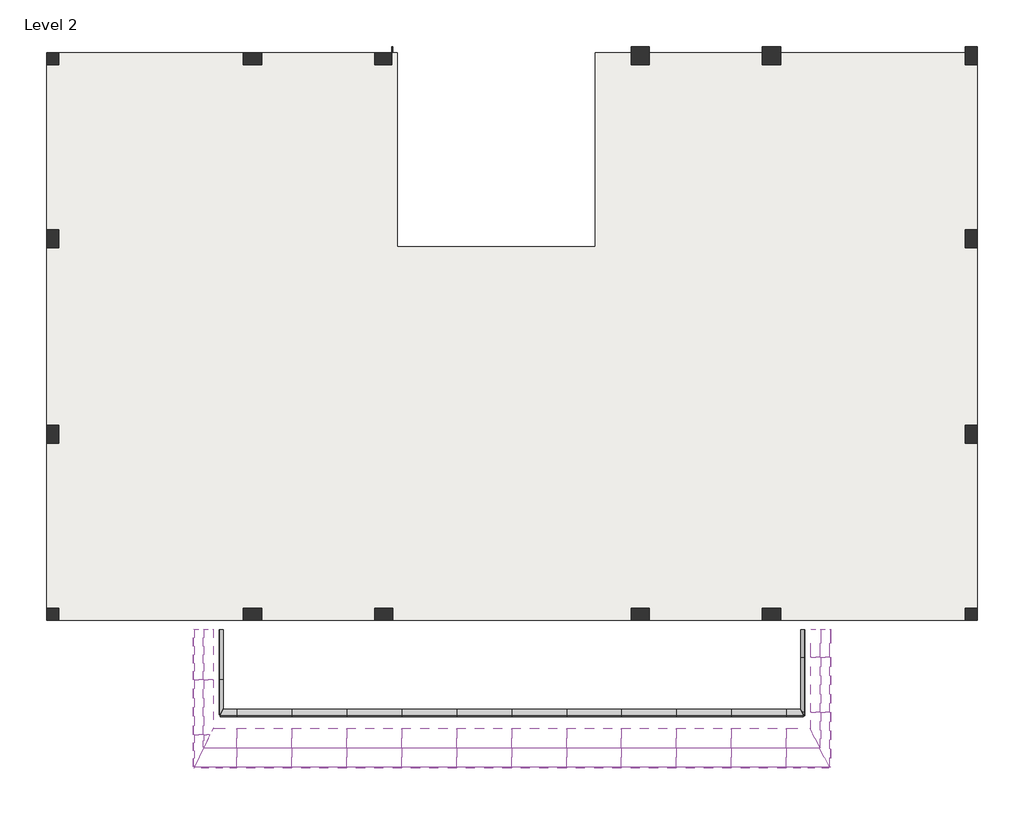
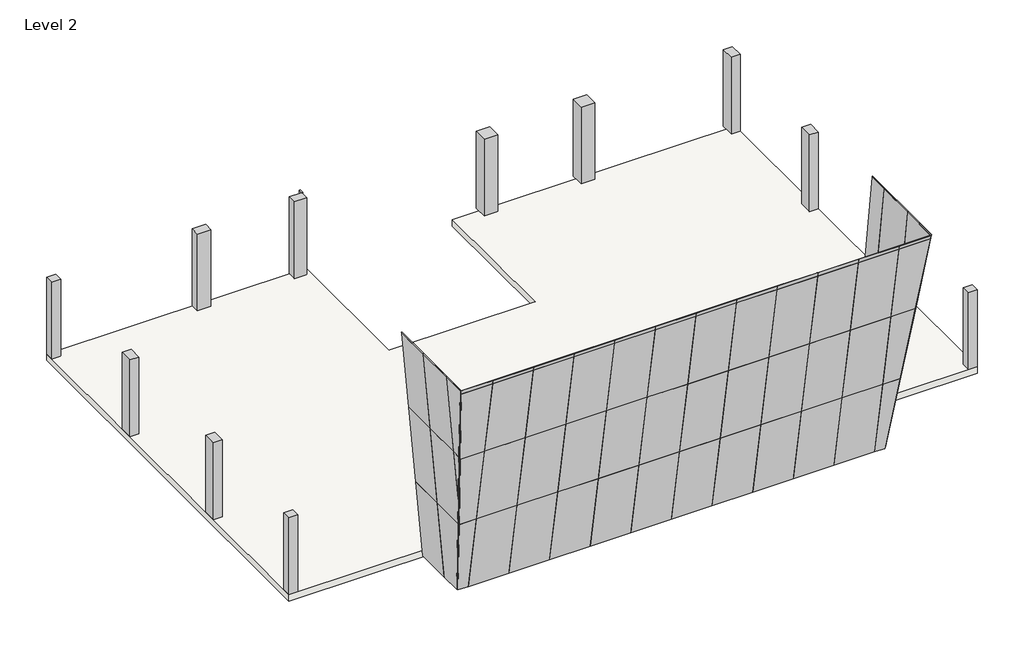
# One storey: 71 plates, 16 columns, 1 slab.
"""IFC4 building model written with IfcOpenShell, lengths in millimetres."""

import ifcopenshell
import ifcopenshell.guid

model = None  # the IFC model being written
_history = None  # IfcOwnerHistory: only IFC2X3 demands one
_inside = {}  # id of a spatial element -> (the spatial element, [elements in it])
_under = {}  # id of a project, library or spatial element -> (it, [spatial elements below it])
_declared = {}  # id of a project -> (the project, [libraries it declares])
_typed = {}  # id of a type object -> (the type object, [elements of that type])
_made_of = {}  # id of a material, layer set ... -> (it, [elements and type objects made of it])


def new_model(schema):
    """Start an empty IFC model of exactly this schema.

    Asked for "IFC4X3", IfcOpenShell would pick the latest addendum, in which some entities
    have other attributes; the version numbers below select the first issue.
    IFC2X3 requires an IfcOwnerHistory on every rooted entity: one is made here for all.
    """
    global model, _history
    if schema == "IFC4X3":
        model = ifcopenshell.file(schema_version=(4, 3, 0, 0))
    else:
        model = ifcopenshell.file(schema=schema)
    _inside.clear()
    _under.clear()
    _declared.clear()
    _typed.clear()
    _made_of.clear()
    _history = None
    if model.schema == "IFC2X3":
        org = make("IfcOrganization", Name="unknown")
        user = make(
            "IfcPersonAndOrganization",
            ThePerson=make("IfcPerson", FamilyName="unknown"),
            TheOrganization=org,
        )
        app = make(
            "IfcApplication",
            ApplicationDeveloper=org,
            Version="unknown",
            ApplicationFullName="unknown",
            ApplicationIdentifier="unknown",
        )
        _history = make(
            "IfcOwnerHistory",
            OwningUser=user,
            OwningApplication=app,
            ChangeAction="ADDED",
            CreationDate=0,
        )
    return model


def make(cls, **values):
    """One entity of the class cls with the attributes given. An attribute that is None is left unset."""
    return model.create_entity(
        cls, **{name: value for name, value in values.items() if value is not None}
    )


def rooted(cls, **values):
    """An entity with a GlobalId (a new one), such as an element, a storey or a relation."""
    return make(cls, GlobalId=ifcopenshell.guid.new(), OwnerHistory=_history, **values)


def si_unit(unit_type, name, prefix=None):
    """IfcSIUnit, for example si_unit("LENGTHUNIT", "METRE", prefix="MILLI")."""
    return make("IfcSIUnit", UnitType=unit_type, Prefix=prefix, Name=name)


def assignment(units):
    """IfcUnitAssignment: the units of a project."""
    return None if units is None else make("IfcUnitAssignment", Units=units)


def point(xyz):
    """IfcCartesianPoint."""
    return None if xyz is None else make("IfcCartesianPoint", Coordinates=xyz)


def direction(xyz):
    """IfcDirection."""
    return None if xyz is None else make("IfcDirection", DirectionRatios=xyz)


def frame(location, z_axis=None, x_axis=None):
    """IfcAxis2Placement3D, a coordinate frame: its origin and axes. An axis left out is left unset."""
    return make(
        "IfcAxis2Placement3D",
        Location=point(location),
        Axis=direction(z_axis),
        RefDirection=direction(x_axis),
    )


def origin():
    """The frame at (0, 0, 0) with its axes left unset."""
    return frame((0.0, 0.0, 0.0))


def origin_with_axes():
    """The frame at (0, 0, 0) with the z axis (0, 0, 1) and the x axis (1, 0, 0) written out."""
    return frame((0.0, 0.0, 0.0), z_axis=(0.0, 0.0, 1.0), x_axis=(1.0, 0.0, 0.0))


def place(relative_to, where):
    """IfcLocalPlacement: puts the frame where relative to a parent placement (None: the world)."""
    return make(
        "IfcLocalPlacement", PlacementRelTo=relative_to, RelativePlacement=where
    )


def context(
    kind, dimensions, precision=None, world=None, true_north=None, identifier=None
):
    """IfcGeometricRepresentationContext, for example the 3D "Model" context."""
    return make(
        "IfcGeometricRepresentationContext",
        ContextIdentifier=identifier,
        ContextType=kind,
        CoordinateSpaceDimension=dimensions,
        Precision=precision,
        WorldCoordinateSystem=world,
        TrueNorth=true_north,
    )


def project(units=None, contexts=None):
    """IfcProject with its units and contexts."""
    return rooted(
        "IfcProject",
        Name="project",
        RepresentationContexts=contexts,
        UnitsInContext=assignment(units),
    )


def spatial(cls, under=None, at=None, **own):
    """A site, building, storey or space (cls), placed at a placement, below another one or the project."""
    s = rooted(cls, ObjectPlacement=at, **own)
    if under is not None:
        _under.setdefault(under.id(), (under, []))[1].append(s)
    return s


def polyline(points):
    """IfcPolyline through the points."""
    return make("IfcPolyline", Points=[point(p) for p in points])


def outline(outer, holes=None, kind="AREA"):
    """IfcArbitraryClosedProfileDef: a profile drawn as a closed curve; with holes, ...WithVoids."""
    if holes is None:
        return make("IfcArbitraryClosedProfileDef", ProfileType=kind, OuterCurve=outer)
    return make(
        "IfcArbitraryProfileDefWithVoids",
        ProfileType=kind,
        OuterCurve=outer,
        InnerCurves=holes,
    )


def extrude(swept, where, along, depth):
    """IfcExtrudedAreaSolid: the profile swept, set in the frame where, extruded along a direction by depth."""
    return make(
        "IfcExtrudedAreaSolid",
        SweptArea=swept,
        Position=where,
        ExtrudedDirection=direction(along),
        Depth=depth,
    )


def shape(context_of_items, identifier, shape_type, items):
    """IfcShapeRepresentation: the items that make up one representation, for example the "Body"."""
    return make(
        "IfcShapeRepresentation",
        ContextOfItems=context_of_items,
        RepresentationIdentifier=identifier,
        RepresentationType=shape_type,
        Items=items,
    )


def source(mapping_origin, context_of_items, identifier, shape_type, items):
    """IfcRepresentationMap: a shape defined once, which mapped items show again and again."""
    return make(
        "IfcRepresentationMap",
        MappingOrigin=mapping_origin,
        MappedRepresentation=shape(context_of_items, identifier, shape_type, items),
    )


def transform(
    local_origin,
    x_axis=None,
    y_axis=None,
    z_axis=None,
    scale=None,
    scale2=None,
    scale3=None,
    uniform=True,
):
    """IfcCartesianTransformationOperator3D, or its non-uniform kind. x_axis, y_axis, z_axis: its Axis1, 2, 3."""
    if uniform:
        return make(
            "IfcCartesianTransformationOperator3D",
            Axis1=direction(x_axis),
            Axis2=direction(y_axis),
            LocalOrigin=point(local_origin),
            Scale=scale,
            Axis3=direction(z_axis),
        )
    return make(
        "IfcCartesianTransformationOperator3DnonUniform",
        Axis1=direction(x_axis),
        Axis2=direction(y_axis),
        LocalOrigin=point(local_origin),
        Scale=scale,
        Axis3=direction(z_axis),
        Scale2=scale2,
        Scale3=scale3,
    )


def mapped(mapping_source, mapping_target):
    """IfcMappedItem: shows the shape of a source again, moved by a transform."""
    return make(
        "IfcMappedItem", MappingSource=mapping_source, MappingTarget=mapping_target
    )


def made_of(thing, what):
    """Note that an element or type object is made of a material, layer set ...; save() writes the relation."""
    if what is not None:
        _made_of.setdefault(what.id(), (what, []))[1].append(thing)
    return thing


def element(
    cls,
    number,
    at=None,
    inside=None,
    cuts=None,
    type_object=None,
    material=None,
    context=None,
    identifier="Body",
    shape_type=None,
    held_by="IfcProductDefinitionShape",
    body=None,
    shapes=None,
    **own,
):
    """One element of the class cls, such as IfcWall. Its Tag is "e" and its number.

    at: its placement. inside: the storey or other place that contains it. cuts: it is an
    opening in that element (IfcRelVoidsElement). A single representation is given by context,
    identifier, shape_type and body (its items); several are given by shapes. held_by: the class
    of the entity that holds the representations. save() writes the other relations.
    """
    e = rooted(cls, Tag="e%d" % number, ObjectPlacement=at, **own)
    if body is not None:
        shapes = [shape(context, identifier, shape_type, body)]
    if shapes is not None:
        e.Representation = make(held_by, Representations=shapes)
    if inside is not None:
        _inside.setdefault(inside.id(), (inside, []))[1].append(e)
    if cuts is not None:
        rooted(
            "IfcRelVoidsElement", RelatingBuildingElement=cuts, RelatedOpeningElement=e
        )
    if type_object is not None:
        _typed.setdefault(type_object.id(), (type_object, []))[1].append(e)
    return made_of(e, material)


def aggregate(whole, parts):
    """IfcRelAggregates: a whole, such as a stair, and the parts it consists of."""
    return rooted("IfcRelAggregates", RelatingObject=whole, RelatedObjects=parts)


def save(model, path):
    """Write the relations noted so far, then the file.

    IfcRelAggregates (storeys below a building ...), IfcRelContainedInSpatialStructure (elements
    in a storey), IfcRelDefinesByType, IfcRelAssociatesMaterial and IfcRelDeclares: one each for
    every whole, place, type object, material and project.
    """
    for whole, parts in _under.values():
        aggregate(whole, parts)
    for where, things in _inside.values():
        rooted(
            "IfcRelContainedInSpatialStructure",
            RelatedElements=things,
            RelatingStructure=where,
        )
    for kind, things in _typed.values():
        rooted("IfcRelDefinesByType", RelatedObjects=things, RelatingType=kind)
    for what, things in _made_of.values():
        rooted("IfcRelAssociatesMaterial", RelatedObjects=things, RelatingMaterial=what)
    for by, libraries in _declared.values():
        rooted("IfcRelDeclares", RelatingContext=by, RelatedDefinitions=libraries)
    model.write(path)


def system_panel_glazed_2e91cb65(model_context):
    return source(origin(), model_context, "Body", "SweptSolid", [
        extrude(outline(polyline([(838.2000002, -44.45), (-838.2000002, -44.45), (-838.2000002, -19.05), (838.2000002, -19.05), (838.2000002, -44.45)])), origin_with_axes(), (0.0, 0.0, 1.0), 3657.6),
    ])


def system_panel_glazed_41c8569a(model_context):
    return source(origin(), model_context, "Body", "SweptSolid", [
        extrude(outline(polyline([(3054.1438606, -268.2393521), (0.0, 268.2393521), (3054.1438606, 268.2393521), (3054.1438606, -268.2393521)])), frame((0.0, -44.45, 0.0), z_axis=(0.0, 1.0, 0.0), x_axis=(0.0, 0.0, 1.0)), (0.0, 0.0, 1.0), 25.4),
    ])


def system_panel_glazed_2bad594a(model_context):
    return source(origin(), model_context, "Body", "SweptSolid", [
        extrude(outline(polyline([(0.0, -797.3917397), (0.0, 154.912342), (3657.6, 797.3917397), (3657.6, -797.3917397), (0.0, -797.3917397)])), frame((0.0, -44.45, 0.0), z_axis=(0.0, 1.0, 0.0), x_axis=(0.0, 0.0, 1.0)), (0.0, 0.0, 1.0), 25.4),
    ])


def system_panel_glazed_87679f4c(model_context):
    return source(origin(), model_context, "Body", "SweptSolid", [
        extrude(outline(polyline([(0.0, -914.4), (0.0, 680.3834794), (1332.2432262, 914.4), (3657.6, 914.4), (3657.6, -914.4), (0.0, -914.4)])), frame((0.0, -44.45, 0.0), z_axis=(0.0, 1.0, 0.0), x_axis=(0.0, 0.0, 1.0)), (0.0, 0.0, 1.0), 25.4),
    ])


def system_panel_glazed_96c5221b(model_context):
    return source(origin(), model_context, "Body", "SweptSolid", [
        extrude(outline(polyline([(0.0, -204.2314386), (2325.3567738, 204.2314386), (2325.3567738, -204.2314386), (0.0, -204.2314386)])), frame((0.0, -44.45, 0.0), z_axis=(0.0, 1.0, 0.0), x_axis=(0.0, 0.0, 1.0)), (0.0, 0.0, 1.0), 25.4),
    ])


def system_panel_glazed_1f34555f(model_context):
    return source(origin(), model_context, "Body", "SweptSolid", [
        extrude(outline(polyline([(914.4, -44.45), (-914.4, -44.45), (-914.4, -19.05), (914.4, -19.05), (914.4, -44.45)])), origin_with_axes(), (0.0, 0.0, 1.0), 3657.6),
    ])


def system_panel_glazed_ce152239(model_context):
    return source(origin(), model_context, "Body", "SweptSolid", [
        extrude(outline(polyline([(0.0, -525.4711374), (0.0, -117.0082603), (3657.6, 525.4711374), (3657.6, -525.4711374), (0.0, -525.4711374)])), frame((0.0, -44.45, 0.0), z_axis=(0.0, 1.0, 0.0), x_axis=(0.0, 0.0, 1.0)), (0.0, 0.0, 1.0), 25.4),
    ])


def system_panel_glazed_8b4ddac8(model_context):
    return source(origin(), model_context, "Body", "SweptSolid", [
        extrude(outline(polyline([(838.2000002, -44.45), (-838.2000002, -44.45), (-838.2000002, -19.05), (838.2000002, -19.05), (838.2000002, -44.45)])), origin_with_axes(), (0.0, 0.0, 1.0), 41.9143134),
    ])


def system_panel_glazed_7f82afe2(model_context):
    return source(origin(), model_context, "Body", "SweptSolid", [
        extrude(outline(polyline([(914.4, -44.45), (-914.4, -44.45), (-914.4, -19.05), (914.4, -19.05), (914.4, -44.45)])), origin_with_axes(), (0.0, 0.0, 1.0), 41.9143134),
    ])


def system_panel_glazed_3146f186(model_context):
    return source(origin(), model_context, "Body", "SweptSolid", [
        extrude(outline(polyline([(0.0, -529.1523878), (0.0, 521.789887), (41.9143134, 529.1523878), (41.9143134, -529.1523878), (0.0, -529.1523878)])), frame((0.0, -44.45, 0.0), z_axis=(0.0, 1.0, 0.0), x_axis=(0.0, 0.0, 1.0)), (0.0, 0.0, 1.0), 25.4),
    ])


def system_panel_glazed_f4345ae3(model_context):
    return source(origin(), model_context, "Body", "SweptSolid", [
        extrude(outline(polyline([(914.4, -44.45), (-914.4, -44.45), (-914.4, -19.05), (914.4, -19.05), (914.4, -44.45)])), origin_with_axes(), (0.0, 0.0, 1.0), 169.2731269),
    ])


def system_panel_glazed_866ab655(model_context):
    return source(origin(), model_context, "Body", "SweptSolid", [
        extrude(outline(polyline([(0.0, -808.3993064), (0.0, 914.4), (3657.6, 914.4), (3657.6, -914.4), (603.4561394, -914.4), (0.0, -808.3993064)])), frame((0.0, -44.45, 0.0), z_axis=(0.0, 1.0, 0.0), x_axis=(0.0, 0.0, 1.0)), (0.0, 0.0, 1.0), 25.4),
    ])


def system_panel_glazed_b062bbc2(model_context):
    return source(origin(), model_context, "Body", "SweptSolid", [
        extrude(outline(polyline([(465.8483058, -44.45), (-465.8483058, -44.45), (-465.8483058, -19.05), (465.8483058, -19.05), (465.8483058, -44.45)])), origin_with_axes(), (0.0, 0.0, 1.0), 3657.6),
    ])


def system_panel_glazed_bcd6892e(model_context):
    return source(origin(), model_context, "Body", "SweptSolid", [
        extrude(outline(polyline([(0.0, 53.0003468), (0.0, 589.4790509), (3657.6, 589.4790509), (3657.6, -589.4790509), (0.0, 53.0003468)])), frame((0.0, -44.45, 0.0), z_axis=(0.0, 1.0, 0.0), x_axis=(0.0, 0.0, 1.0)), (0.0, 0.0, 1.0), 25.4),
    ])


def system_panel_glazed_e7bd2299(model_context):
    return source(origin(), model_context, "Body", "SweptSolid", [
        extrude(outline(polyline([(0.0, -268.2393521), (0.0, 910.7187498), (3657.6, 910.7187498), (3657.6, -910.7187498), (0.0, -268.2393521)])), frame((0.0, -44.45, 0.0), z_axis=(0.0, 1.0, 0.0), x_axis=(0.0, 0.0, 1.0)), (0.0, 0.0, 1.0), 25.4),
    ])


def system_panel_glazed_0a43eb3e(model_context):
    return source(origin(), model_context, "Body", "SweptSolid", [
        extrude(outline(polyline([(0.0, -907.0374994), (0.0, 914.4000002), (41.9143134, 914.4000002), (41.9143134, -914.4000002), (0.0, -907.0374994)])), frame((0.0, -44.45, 0.0), z_axis=(0.0, 1.0, 0.0), x_axis=(0.0, 0.0, 1.0)), (0.0, 0.0, 1.0), 25.4),
    ])


def system_panel_glazed_c48c36d0(model_context):
    return source(origin(), model_context, "Body", "SweptSolid", [
        extrude(outline(polyline([(465.8483058, -44.45), (-465.8483058, -44.45), (-465.8483058, -19.05), (465.8483058, -19.05), (465.8483058, -44.45)])), origin_with_axes(), (0.0, 0.0, 1.0), 41.9143134),
    ])


def system_panel_glazed_35afb83b(model_context):
    return source(origin(), model_context, "Body", "SweptSolid", [
        extrude(outline(polyline([(0.0, -71.0314805), (0.0, 386.1685195), (3657.6, 386.1685195), (3657.6, -386.1685195), (0.0, -71.0314805)])), frame((0.0, -44.45, 0.0), z_axis=(0.0, 1.0, 0.0), x_axis=(0.0, 0.0, 1.0)), (0.0, 0.0, 1.0), 25.4),
    ])


def system_panel_glazed_ca25d662(model_context):
    return source(origin(), model_context, "Body", "SweptSolid", [
        extrude(outline(polyline([(0.0, -386.1685195), (0.0, 71.0314805), (3657.6, 386.1685195), (3657.6, -386.1685195), (0.0, -386.1685195)])), frame((0.0, -44.45, 0.0), z_axis=(0.0, 1.0, 0.0), x_axis=(0.0, 0.0, 1.0)), (0.0, 0.0, 1.0), 25.4),
    ])


def system_panel_glazed_d5b9b34d(model_context):
    return source(origin(), model_context, "Body", "SweptSolid", [
        extrude(outline(polyline([(0.0, -228.6), (0.0, 543.7370389), (3657.6, 543.7370389), (3657.6, -543.7370389), (0.0, -228.6)])), frame((0.0, -44.45, 0.0), z_axis=(0.0, 1.0, 0.0), x_axis=(0.0, 0.0, 1.0)), (0.0, 0.0, 1.0), 25.4),
    ])


def system_panel_glazed_127879aa(model_context):
    return source(origin(), model_context, "Body", "SweptSolid", [
        extrude(outline(polyline([(0.0, -543.7370389), (0.0, 228.6), (3657.6, 543.7370389), (3657.6, -543.7370389), (0.0, -543.7370389)])), frame((0.0, -44.45, 0.0), z_axis=(0.0, 1.0, 0.0), x_axis=(0.0, 0.0, 1.0)), (0.0, 0.0, 1.0), 25.4),
    ])


def system_panel_glazed_cde5e94a(model_context):
    return source(origin(), model_context, "Body", "SweptSolid", [
        extrude(outline(polyline([(0.0, -386.1685195), (0.0, 701.3055584), (3657.6, 701.3055584), (3657.6, -701.3055584), (0.0, -386.1685195)])), frame((0.0, -44.45, 0.0), z_axis=(0.0, 1.0, 0.0), x_axis=(0.0, 0.0, 1.0)), (0.0, 0.0, 1.0), 25.4),
    ])


def system_panel_glazed_b3fa7013(model_context):
    return source(origin(), model_context, "Body", "SweptSolid", [
        extrude(outline(polyline([(0.0, -701.3055584), (0.0, 386.1685195), (3657.6, 701.3055584), (3657.6, -701.3055584), (0.0, -701.3055584)])), frame((0.0, -44.45, 0.0), z_axis=(0.0, 1.0, 0.0), x_axis=(0.0, 0.0, 1.0)), (0.0, 0.0, 1.0), 25.4),
    ])


def system_panel_glazed_d86b06c2(model_context):
    return source(origin(), model_context, "Body", "SweptSolid", [
        extrude(outline(polyline([(0.0, -694.0133132), (0.0, 708.5978036), (169.2731269, 708.5978036), (169.2731269, -708.5978036), (0.0, -694.0133132)])), frame((0.0, -44.45, 0.0), z_axis=(0.0, 1.0, 0.0), x_axis=(0.0, 0.0, 1.0)), (0.0, 0.0, 1.0), 25.4),
    ])


def system_panel_glazed_9c30f1a4(model_context):
    return source(origin(), model_context, "Body", "SweptSolid", [
        extrude(outline(polyline([(0.0, -708.5978036), (0.0, 694.0133132), (169.2731269, 708.5978036), (169.2731269, -708.5978036), (0.0, -708.5978036)])), frame((0.0, -44.45, 0.0), z_axis=(0.0, 1.0, 0.0), x_axis=(0.0, 0.0, 1.0)), (0.0, 0.0, 1.0), 25.4),
    ])


model = new_model("IFC4")

# Units and contexts
model_context = context("Model", 3, world=origin())
ifc_project = project(units=[si_unit("LENGTHUNIT", "METRE", prefix="MILLI")], contexts=[model_context])

# Site, building, storey
site = spatial("IfcSite", under=ifc_project)
building = spatial("IfcBuilding", under=site)
storey = spatial("IfcBuildingStorey", under=building, Name="Level 2", Elevation=3657.6)

# Columns
placement = place(None, origin())
element("IfcColumn", 1, ObjectType="Rectangular Column : 24\" x 24\"", at=placement, inside=storey, context=model_context, shape_type="SweptSolid", body=[
    extrude(outline(polyline([(-16253.4122732, 9291.5015304), (-16253.4122732, 8885.1015304), (-16659.8122732, 8885.1015304), (-16659.8122732, 9291.5015304), (-16253.4122732, 9291.5015304)])), frame((0.0, 0.0, 3657.6), z_axis=(0.0, 0.0, 1.0), x_axis=(1.0, 0.0, 0.0)), (0.0, 0.0, 1.0), 3657.6),
])
element("IfcColumn", 2, ObjectType="Rectangular Column : 24\" x 24\"", at=placement, inside=storey, context=model_context, shape_type="SweptSolid", body=[
    extrude(outline(polyline([(-16253.4122732, 3398.7015304), (-16253.4122732, 2789.1015304), (-16659.8122732, 2789.1015304), (-16659.8122732, 3398.7015304), (-16253.4122732, 3398.7015304)])), frame((0.0, 0.0, 3657.6), z_axis=(0.0, 0.0, 1.0), x_axis=(1.0, 0.0, 0.0)), (0.0, 0.0, 1.0), 3657.6),
])
element("IfcColumn", 3, ObjectType="Rectangular Column : 24\" x 24\"", at=placement, inside=storey, context=model_context, shape_type="SweptSolid", body=[
    extrude(outline(polyline([(-9497.0122732, 8885.1015304), (-10106.6122732, 8885.1015304), (-10106.6122732, 9291.5015304), (-9497.0122732, 9291.5015304), (-9497.0122732, 8885.1015304)])), frame((0.0, 0.0, 3657.6), z_axis=(0.0, 0.0, 1.0), x_axis=(1.0, 0.0, 0.0)), (0.0, 0.0, 1.0), 3657.6),
])
element("IfcColumn", 4, ObjectType="Rectangular Column : 24\" x 24\"", at=placement, inside=storey, context=model_context, shape_type="SweptSolid", body=[
    extrude(outline(polyline([(-5174.2497732, 9494.7015304), (-5128.2122732, 9494.7015304), (-5128.2122732, 9301.0265304), (-5174.2497732, 9301.0265304), (-5174.2497732, 9494.7015304)])), frame((0.0, 0.0, 3657.6), z_axis=(0.0, 0.0, 1.0), x_axis=(1.0, 0.0, 0.0)), (0.0, 0.0, 1.0), 3657.6),
    extrude(outline(polyline([(-5737.8122732, 8885.1015304), (-5737.8122732, 9291.5015304), (-5174.2497732, 9291.5015304), (-5174.2497732, 8885.1015304), (-5737.8122732, 8885.1015304)])), frame((0.0, 0.0, 3657.6), z_axis=(0.0, 0.0, 1.0), x_axis=(1.0, 0.0, 0.0)), (0.0, 0.0, 1.0), 3657.6),
])
element("IfcColumn", 5, ObjectType="Rectangular Column : 24\" x 24\"", at=placement, inside=storey, context=model_context, shape_type="SweptSolid", body=[
    extrude(outline(polyline([(3406.1877268, 9494.7015304), (3406.1877268, 8885.1015304), (2796.5877268, 8885.1015304), (2796.5877268, 9494.7015304), (3406.1877268, 9494.7015304)])), frame((0.0, 0.0, 3657.6), z_axis=(0.0, 0.0, 1.0), x_axis=(1.0, 0.0, 0.0)), (0.0, 0.0, 1.0), 3657.6),
])
element("IfcColumn", 6, ObjectType="Rectangular Column : 24\" x 24\"", at=placement, inside=storey, context=model_context, shape_type="SweptSolid", body=[
    extrude(outline(polyline([(7774.9877268, 9494.7015304), (7774.9877268, 8885.1015304), (7165.3877268, 8885.1015304), (7165.3877268, 9494.7015304), (7774.9877268, 9494.7015304)])), frame((0.0, 0.0, 3657.6), z_axis=(0.0, 0.0, 1.0), x_axis=(1.0, 0.0, 0.0)), (0.0, 0.0, 1.0), 3657.6),
])
element("IfcColumn", 7, ObjectType="Rectangular Column : 24\" x 24\"", at=placement, inside=storey, context=model_context, shape_type="SweptSolid", body=[
    extrude(outline(polyline([(13921.7877268, 8885.1015304), (13921.7877268, 9494.7015304), (14328.1877268, 9494.7015304), (14328.1877268, 8885.1015304), (13921.7877268, 8885.1015304)])), frame((0.0, 0.0, 3657.6), z_axis=(0.0, 0.0, 1.0), x_axis=(1.0, 0.0, 0.0)), (0.0, 0.0, 1.0), 3657.6),
])
element("IfcColumn", 8, ObjectType="Rectangular Column : 24\" x 24\"", at=placement, inside=storey, context=model_context, shape_type="SweptSolid", body=[
    extrude(outline(polyline([(13921.7877268, 2789.1015304), (13921.7877268, 3398.7015304), (14328.1877268, 3398.7015304), (14328.1877268, 2789.1015304), (13921.7877268, 2789.1015304)])), frame((0.0, 0.0, 3657.6), z_axis=(0.0, 0.0, 1.0), x_axis=(1.0, 0.0, 0.0)), (0.0, 0.0, 1.0), 3657.6),
])
element("IfcColumn", 9, ObjectType="Rectangular Column : 24\" x 24\"", at=placement, inside=storey, context=model_context, shape_type="SweptSolid", body=[
    extrude(outline(polyline([(13921.7877268, -3713.2984696), (13921.7877268, -3103.6984696), (14328.1877268, -3103.6984696), (14328.1877268, -3713.2984696), (13921.7877268, -3713.2984696)])), frame((0.0, 0.0, 3657.6), z_axis=(0.0, 0.0, 1.0), x_axis=(1.0, 0.0, 0.0)), (0.0, 0.0, 1.0), 3657.6),
])
element("IfcColumn", 10, ObjectType="Rectangular Column : 24\" x 24\"", at=placement, inside=storey, context=model_context, shape_type="SweptSolid", body=[
    extrude(outline(polyline([(13921.7877268, -9606.0984696), (13921.7877268, -9199.6984696), (14328.1877268, -9199.6984696), (14328.1877268, -9606.0984696), (13921.7877268, -9606.0984696)])), frame((0.0, 0.0, 3657.6), z_axis=(0.0, 0.0, 1.0), x_axis=(1.0, 0.0, 0.0)), (0.0, 0.0, 1.0), 3657.6),
])
element("IfcColumn", 11, ObjectType="Rectangular Column : 24\" x 24\"", at=placement, inside=storey, context=model_context, shape_type="SweptSolid", body=[
    extrude(outline(polyline([(7165.3877268, -9199.6984696), (7774.9877268, -9199.6984696), (7774.9877268, -9606.0984696), (7165.3877268, -9606.0984696), (7165.3877268, -9199.6984696)])), frame((0.0, 0.0, 3657.6), z_axis=(0.0, 0.0, 1.0), x_axis=(1.0, 0.0, 0.0)), (0.0, 0.0, 1.0), 3657.6),
])
element("IfcColumn", 12, ObjectType="Rectangular Column : 24\" x 24\"", at=placement, inside=storey, context=model_context, shape_type="SweptSolid", body=[
    extrude(outline(polyline([(2796.5877268, -9199.6984696), (3406.1877268, -9199.6984696), (3406.1877268, -9606.0984696), (2796.5877268, -9606.0984696), (2796.5877268, -9199.6984696)])), frame((0.0, 0.0, 3657.6), z_axis=(0.0, 0.0, 1.0), x_axis=(1.0, 0.0, 0.0)), (0.0, 0.0, 1.0), 3657.6),
])
element("IfcColumn", 13, ObjectType="Rectangular Column : 24\" x 24\"", at=placement, inside=storey, context=model_context, shape_type="SweptSolid", body=[
    extrude(outline(polyline([(-5737.8122732, -9199.6984696), (-5128.2122732, -9199.6984696), (-5128.2122732, -9606.0984696), (-5737.8122732, -9606.0984696), (-5737.8122732, -9199.6984696)])), frame((0.0, 0.0, 3657.6), z_axis=(0.0, 0.0, 1.0), x_axis=(1.0, 0.0, 0.0)), (0.0, 0.0, 1.0), 3657.6),
])
element("IfcColumn", 14, ObjectType="Rectangular Column : 24\" x 24\"", at=placement, inside=storey, context=model_context, shape_type="SweptSolid", body=[
    extrude(outline(polyline([(-10106.6122732, -9199.6984696), (-9497.0122732, -9199.6984696), (-9497.0122732, -9606.0984696), (-10106.6122732, -9606.0984696), (-10106.6122732, -9199.6984696)])), frame((0.0, 0.0, 3657.6), z_axis=(0.0, 0.0, 1.0), x_axis=(1.0, 0.0, 0.0)), (0.0, 0.0, 1.0), 3657.6),
])
element("IfcColumn", 15, ObjectType="Rectangular Column : 24\" x 24\"", at=placement, inside=storey, context=model_context, shape_type="SweptSolid", body=[
    extrude(outline(polyline([(-16659.8122732, -9199.6984696), (-16253.4122732, -9199.6984696), (-16253.4122732, -9606.0984696), (-16659.8122732, -9606.0984696), (-16659.8122732, -9199.6984696)])), frame((0.0, 0.0, 3657.6), z_axis=(0.0, 0.0, 1.0), x_axis=(1.0, 0.0, 0.0)), (0.0, 0.0, 1.0), 3657.6),
])
element("IfcColumn", 16, ObjectType="Rectangular Column : 24\" x 24\"", at=placement, inside=storey, context=model_context, shape_type="SweptSolid", body=[
    extrude(outline(polyline([(-16253.4122732, -3103.6984696), (-16253.4122732, -3713.2984696), (-16659.8122732, -3713.2984696), (-16659.8122732, -3103.6984696), (-16253.4122732, -3103.6984696)])), frame((0.0, 0.0, 3657.6), z_axis=(0.0, 0.0, 1.0), x_axis=(1.0, 0.0, 0.0)), (0.0, 0.0, 1.0), 3657.6),
])

# Plates
system_panel_glazed_shape = system_panel_glazed_2e91cb65(model_context)
element("IfcPlate", 17, ObjectType="System Panel : Glazed", at=placement, inside=storey, context=model_context, shape_type="MappedRepresentation", body=[
    mapped(system_panel_glazed_shape, transform((-10766.9154339, -10749.0984697, 3656.4931221), x_axis=(0.0, -1.0, 0.0), y_axis=(0.9961946980917455, 0.0, 0.08715574274765803), z_axis=(-0.08715574274765803, 0.0, 0.9961946980917455))),
])
element("IfcPlate", 18, ObjectType="System Panel : Glazed", at=placement, inside=storey, context=model_context, shape_type="MappedRepresentation", body=[
    mapped(system_panel_glazed_shape, transform((-11085.6962786, -10749.0984697, 7300.1748498), x_axis=(0.0, -1.0, 0.0), y_axis=(0.9961946980917455, 0.0, 0.08715574274765803), z_axis=(-0.08715574274765803, 0.0, 0.9961946980917455))),
])
element("IfcPlate", 19, ObjectType="System Panel : Glazed", at=placement, inside=storey, context=model_context, shape_type="MappedRepresentation", body=[
    mapped(system_panel_glazed_shape, transform((-11404.4771233, -10749.0984697, 10943.8565775), x_axis=(0.0, -1.0, 0.0), y_axis=(0.9961946980917455, 0.0, 0.08715574274765803), z_axis=(-0.08715574274765803, 0.0, 0.9961946980917455))),
])
system_panel_glazed_2_shape = system_panel_glazed_41c8569a(model_context)
element("IfcPlate", 20, ObjectType="System Panel : Glazed", at=placement, inside=storey, context=model_context, shape_type="MappedRepresentation", body=[
    mapped(system_panel_glazed_2_shape, transform((8487.8855556, -12939.6344332, 4257.6529286), x_axis=(0.0, 1.0, 0.0), y_axis=(-0.9961946980917455, 0.0, 0.08715574274765803), z_axis=(0.08715574274765803, 0.0, 0.9961946980917455))),
])
system_panel_glazed_3_shape = system_panel_glazed_2bad594a(model_context)
element("IfcPlate", 21, ObjectType="System Panel : Glazed", at=placement, inside=storey, context=model_context, shape_type="MappedRepresentation", body=[
    mapped(system_panel_glazed_3_shape, transform((-10766.9154339, -12384.6902096, 3656.4931221), x_axis=(0.0, -1.0, 0.0), y_axis=(0.9961946980917455, 0.0, 0.08715574274765803), z_axis=(-0.08715574274765803, 0.0, 0.9961946980917455))),
])
system_panel_glazed_4_shape = system_panel_glazed_87679f4c(model_context)
element("IfcPlate", 22, ObjectType="System Panel : Glazed", at=placement, inside=storey, context=model_context, shape_type="MappedRepresentation", body=[
    mapped(system_panel_glazed_4_shape, transform((-11085.6962786, -12501.6984699, 7300.1748498), x_axis=(0.0, -1.0, 0.0), y_axis=(0.9961946980917455, 0.0, 0.08715574274765803), z_axis=(-0.08715574274765803, 0.0, 0.9961946980917455))),
])
system_panel_glazed_5_shape = system_panel_glazed_96c5221b(model_context)
element("IfcPlate", 23, ObjectType="System Panel : Glazed", at=placement, inside=storey, context=model_context, shape_type="MappedRepresentation", body=[
    mapped(system_panel_glazed_5_shape, transform((-11201.8089265, -13620.3299085, 8627.3484884), x_axis=(0.0, -1.0, 0.0), y_axis=(0.9961946980917455, 0.0, 0.08715574274765803), z_axis=(-0.08715574274765803, 0.0, 0.9961946980917455))),
])
system_panel_glazed_6_shape = system_panel_glazed_1f34555f(model_context)
element("IfcPlate", 24, ObjectType="System Panel : Glazed", at=placement, inside=storey, context=model_context, shape_type="MappedRepresentation", body=[
    mapped(system_panel_glazed_6_shape, transform((-11404.4771233, -12501.6984699, 10943.8565775), x_axis=(0.0, -1.0, 0.0), y_axis=(0.9961946980917455, 0.0, 0.08715574274765803), z_axis=(-0.08715574274765803, 0.0, 0.9961946980917455))),
])
element("IfcPlate", 25, ObjectType="System Panel : Glazed", at=placement, inside=storey, context=model_context, shape_type="MappedRepresentation", body=[
    mapped(system_panel_glazed_6_shape, transform((-9408.1607851, -12552.1096101, 3655.3946681), x_axis=(1.0, 0.0, 0.0), y_axis=(0.0, 0.9848077530122081, 0.17364817766693014), z_axis=(0.0, -0.17364817766693014, 0.9848077530122081))),
])
element("IfcPlate", 26, ObjectType="System Panel : Glazed", at=placement, inside=storey, context=model_context, shape_type="MappedRepresentation", body=[
    mapped(system_panel_glazed_6_shape, transform((-7579.3607851, -12552.1096101, 3655.3946681), x_axis=(1.0, 0.0, 0.0), y_axis=(0.0, 0.9848077530122081, 0.17364817766693014), z_axis=(0.0, -0.17364817766693014, 0.9848077530122081))),
])
element("IfcPlate", 27, ObjectType="System Panel : Glazed", at=placement, inside=storey, context=model_context, shape_type="MappedRepresentation", body=[
    mapped(system_panel_glazed_6_shape, transform((-5750.5607851, -12552.1096101, 3655.3946681), x_axis=(1.0, 0.0, 0.0), y_axis=(0.0, 0.9848077530122081, 0.17364817766693014), z_axis=(0.0, -0.17364817766693014, 0.9848077530122081))),
])
element("IfcPlate", 28, ObjectType="System Panel : Glazed", at=placement, inside=storey, context=model_context, shape_type="MappedRepresentation", body=[
    mapped(system_panel_glazed_6_shape, transform((-3921.7607851, -12552.1096101, 3655.3946681), x_axis=(1.0, 0.0, 0.0), y_axis=(0.0, 0.9848077530122081, 0.17364817766693014), z_axis=(0.0, -0.17364817766693014, 0.9848077530122081))),
])
element("IfcPlate", 29, ObjectType="System Panel : Glazed", at=placement, inside=storey, context=model_context, shape_type="MappedRepresentation", body=[
    mapped(system_panel_glazed_6_shape, transform((-2092.9607851, -12552.1096101, 3655.3946681), x_axis=(1.0, 0.0, 0.0), y_axis=(0.0, 0.9848077530122081, 0.17364817766693014), z_axis=(0.0, -0.17364817766693014, 0.9848077530122081))),
])
element("IfcPlate", 30, ObjectType="System Panel : Glazed", at=placement, inside=storey, context=model_context, shape_type="MappedRepresentation", body=[
    mapped(system_panel_glazed_6_shape, transform((-264.1607851, -12552.1096101, 3655.3946681), x_axis=(1.0, 0.0, 0.0), y_axis=(0.0, 0.9848077530122081, 0.17364817766693014), z_axis=(0.0, -0.17364817766693014, 0.9848077530122081))),
])
element("IfcPlate", 31, ObjectType="System Panel : Glazed", at=placement, inside=storey, context=model_context, shape_type="MappedRepresentation", body=[
    mapped(system_panel_glazed_6_shape, transform((1564.6392149, -12552.1096101, 3655.3946681), x_axis=(1.0, 0.0, 0.0), y_axis=(0.0, 0.9848077530122081, 0.17364817766693014), z_axis=(0.0, -0.17364817766693014, 0.9848077530122081))),
])
element("IfcPlate", 32, ObjectType="System Panel : Glazed", at=placement, inside=storey, context=model_context, shape_type="MappedRepresentation", body=[
    mapped(system_panel_glazed_6_shape, transform((3393.4392149, -12552.1096101, 3655.3946681), x_axis=(1.0, 0.0, 0.0), y_axis=(0.0, 0.9848077530122081, 0.17364817766693014), z_axis=(0.0, -0.17364817766693014, 0.9848077530122081))),
])
element("IfcPlate", 33, ObjectType="System Panel : Glazed", at=placement, inside=storey, context=model_context, shape_type="MappedRepresentation", body=[
    mapped(system_panel_glazed_6_shape, transform((5222.2392149, -12552.1096101, 3655.3946681), x_axis=(1.0, 0.0, 0.0), y_axis=(0.0, 0.9848077530122081, 0.17364817766693014), z_axis=(0.0, -0.17364817766693014, 0.9848077530122081))),
])
element("IfcPlate", 34, ObjectType="System Panel : Glazed", at=placement, inside=storey, context=model_context, shape_type="MappedRepresentation", body=[
    mapped(system_panel_glazed_6_shape, transform((7051.0392149, -12552.1096101, 3655.3946681), x_axis=(1.0, 0.0, 0.0), y_axis=(0.0, 0.9848077530122081, 0.17364817766693014), z_axis=(0.0, -0.17364817766693014, 0.9848077530122081))),
])
element("IfcPlate", 35, ObjectType="System Panel : Glazed", at=placement, inside=storey, context=model_context, shape_type="MappedRepresentation", body=[
    mapped(system_panel_glazed_6_shape, transform((-9408.1607851, -13187.2451847, 7257.4275056), x_axis=(1.0, 0.0, 0.0), y_axis=(0.0, 0.9848077530122081, 0.17364817766693014), z_axis=(0.0, -0.17364817766693014, 0.9848077530122081))),
])
element("IfcPlate", 36, ObjectType="System Panel : Glazed", at=placement, inside=storey, context=model_context, shape_type="MappedRepresentation", body=[
    mapped(system_panel_glazed_6_shape, transform((-7579.3607851, -13187.2451847, 7257.4275056), x_axis=(1.0, 0.0, 0.0), y_axis=(0.0, 0.9848077530122081, 0.17364817766693014), z_axis=(0.0, -0.17364817766693014, 0.9848077530122081))),
])
element("IfcPlate", 37, ObjectType="System Panel : Glazed", at=placement, inside=storey, context=model_context, shape_type="MappedRepresentation", body=[
    mapped(system_panel_glazed_6_shape, transform((-5750.5607851, -13187.2451847, 7257.4275056), x_axis=(1.0, 0.0, 0.0), y_axis=(0.0, 0.9848077530122081, 0.17364817766693014), z_axis=(0.0, -0.17364817766693014, 0.9848077530122081))),
])
element("IfcPlate", 38, ObjectType="System Panel : Glazed", at=placement, inside=storey, context=model_context, shape_type="MappedRepresentation", body=[
    mapped(system_panel_glazed_6_shape, transform((-3921.7607851, -13187.2451847, 7257.4275056), x_axis=(1.0, 0.0, 0.0), y_axis=(0.0, 0.9848077530122081, 0.17364817766693014), z_axis=(0.0, -0.17364817766693014, 0.9848077530122081))),
])
element("IfcPlate", 39, ObjectType="System Panel : Glazed", at=placement, inside=storey, context=model_context, shape_type="MappedRepresentation", body=[
    mapped(system_panel_glazed_6_shape, transform((-2092.9607851, -13187.2451847, 7257.4275056), x_axis=(1.0, 0.0, 0.0), y_axis=(0.0, 0.9848077530122081, 0.17364817766693014), z_axis=(0.0, -0.17364817766693014, 0.9848077530122081))),
])
element("IfcPlate", 40, ObjectType="System Panel : Glazed", at=placement, inside=storey, context=model_context, shape_type="MappedRepresentation", body=[
    mapped(system_panel_glazed_6_shape, transform((-264.1607851, -13187.2451847, 7257.4275056), x_axis=(1.0, 0.0, 0.0), y_axis=(0.0, 0.9848077530122081, 0.17364817766693014), z_axis=(0.0, -0.17364817766693014, 0.9848077530122081))),
])
element("IfcPlate", 41, ObjectType="System Panel : Glazed", at=placement, inside=storey, context=model_context, shape_type="MappedRepresentation", body=[
    mapped(system_panel_glazed_6_shape, transform((1564.6392149, -13187.2451847, 7257.4275056), x_axis=(1.0, 0.0, 0.0), y_axis=(0.0, 0.9848077530122081, 0.17364817766693014), z_axis=(0.0, -0.17364817766693014, 0.9848077530122081))),
])
element("IfcPlate", 42, ObjectType="System Panel : Glazed", at=placement, inside=storey, context=model_context, shape_type="MappedRepresentation", body=[
    mapped(system_panel_glazed_6_shape, transform((3393.4392149, -13187.2451847, 7257.4275056), x_axis=(1.0, 0.0, 0.0), y_axis=(0.0, 0.9848077530122081, 0.17364817766693014), z_axis=(0.0, -0.17364817766693014, 0.9848077530122081))),
])
element("IfcPlate", 43, ObjectType="System Panel : Glazed", at=placement, inside=storey, context=model_context, shape_type="MappedRepresentation", body=[
    mapped(system_panel_glazed_6_shape, transform((5222.2392149, -13187.2451847, 7257.4275056), x_axis=(1.0, 0.0, 0.0), y_axis=(0.0, 0.9848077530122081, 0.17364817766693014), z_axis=(0.0, -0.17364817766693014, 0.9848077530122081))),
])
element("IfcPlate", 44, ObjectType="System Panel : Glazed", at=placement, inside=storey, context=model_context, shape_type="MappedRepresentation", body=[
    mapped(system_panel_glazed_6_shape, transform((7051.0392149, -13187.2451847, 7257.4275056), x_axis=(1.0, 0.0, 0.0), y_axis=(0.0, 0.9848077530122081, 0.17364817766693014), z_axis=(0.0, -0.17364817766693014, 0.9848077530122081))),
])
element("IfcPlate", 45, ObjectType="System Panel : Glazed", at=placement, inside=storey, context=model_context, shape_type="MappedRepresentation", body=[
    mapped(system_panel_glazed_6_shape, transform((-9408.1607851, -13822.3807593, 10859.460343), x_axis=(1.0, 0.0, 0.0), y_axis=(0.0, 0.9848077530122081, 0.17364817766693014), z_axis=(0.0, -0.17364817766693014, 0.9848077530122081))),
])
element("IfcPlate", 46, ObjectType="System Panel : Glazed", at=placement, inside=storey, context=model_context, shape_type="MappedRepresentation", body=[
    mapped(system_panel_glazed_6_shape, transform((-7579.3607851, -13822.3807593, 10859.460343), x_axis=(1.0, 0.0, 0.0), y_axis=(0.0, 0.9848077530122081, 0.17364817766693014), z_axis=(0.0, -0.17364817766693014, 0.9848077530122081))),
])
element("IfcPlate", 47, ObjectType="System Panel : Glazed", at=placement, inside=storey, context=model_context, shape_type="MappedRepresentation", body=[
    mapped(system_panel_glazed_6_shape, transform((-5750.5607851, -13822.3807593, 10859.460343), x_axis=(1.0, 0.0, 0.0), y_axis=(0.0, 0.9848077530122081, 0.17364817766693014), z_axis=(0.0, -0.17364817766693014, 0.9848077530122081))),
])
element("IfcPlate", 48, ObjectType="System Panel : Glazed", at=placement, inside=storey, context=model_context, shape_type="MappedRepresentation", body=[
    mapped(system_panel_glazed_6_shape, transform((-3921.7607851, -13822.3807593, 10859.460343), x_axis=(1.0, 0.0, 0.0), y_axis=(0.0, 0.9848077530122081, 0.17364817766693014), z_axis=(0.0, -0.17364817766693014, 0.9848077530122081))),
])
element("IfcPlate", 49, ObjectType="System Panel : Glazed", at=placement, inside=storey, context=model_context, shape_type="MappedRepresentation", body=[
    mapped(system_panel_glazed_6_shape, transform((-2092.9607851, -13822.3807593, 10859.460343), x_axis=(1.0, 0.0, 0.0), y_axis=(0.0, 0.9848077530122081, 0.17364817766693014), z_axis=(0.0, -0.17364817766693014, 0.9848077530122081))),
])
element("IfcPlate", 50, ObjectType="System Panel : Glazed", at=placement, inside=storey, context=model_context, shape_type="MappedRepresentation", body=[
    mapped(system_panel_glazed_6_shape, transform((-264.1607851, -13822.3807593, 10859.460343), x_axis=(1.0, 0.0, 0.0), y_axis=(0.0, 0.9848077530122081, 0.17364817766693014), z_axis=(0.0, -0.17364817766693014, 0.9848077530122081))),
])
element("IfcPlate", 51, ObjectType="System Panel : Glazed", at=placement, inside=storey, context=model_context, shape_type="MappedRepresentation", body=[
    mapped(system_panel_glazed_6_shape, transform((1564.6392149, -13822.3807593, 10859.460343), x_axis=(1.0, 0.0, 0.0), y_axis=(0.0, 0.9848077530122081, 0.17364817766693014), z_axis=(0.0, -0.17364817766693014, 0.9848077530122081))),
])
element("IfcPlate", 52, ObjectType="System Panel : Glazed", at=placement, inside=storey, context=model_context, shape_type="MappedRepresentation", body=[
    mapped(system_panel_glazed_6_shape, transform((3393.4392149, -13822.3807593, 10859.460343), x_axis=(1.0, 0.0, 0.0), y_axis=(0.0, 0.9848077530122081, 0.17364817766693014), z_axis=(0.0, -0.17364817766693014, 0.9848077530122081))),
])
element("IfcPlate", 53, ObjectType="System Panel : Glazed", at=placement, inside=storey, context=model_context, shape_type="MappedRepresentation", body=[
    mapped(system_panel_glazed_6_shape, transform((5222.2392149, -13822.3807593, 10859.460343), x_axis=(1.0, 0.0, 0.0), y_axis=(0.0, 0.9848077530122081, 0.17364817766693014), z_axis=(0.0, -0.17364817766693014, 0.9848077530122081))),
])
element("IfcPlate", 54, ObjectType="System Panel : Glazed", at=placement, inside=storey, context=model_context, shape_type="MappedRepresentation", body=[
    mapped(system_panel_glazed_6_shape, transform((7051.0392149, -13822.3807593, 10859.460343), x_axis=(1.0, 0.0, 0.0), y_axis=(0.0, 0.9848077530122081, 0.17364817766693014), z_axis=(0.0, -0.17364817766693014, 0.9848077530122081))),
])
element("IfcPlate", 55, ObjectType="System Panel : Glazed", at=placement, inside=storey, context=model_context, shape_type="MappedRepresentation", body=[
    mapped(system_panel_glazed_6_shape, transform((8754.0717322, -11756.9950812, 7300.1748498), x_axis=(0.0, 1.0, 0.0), y_axis=(-0.9961946980917455, 0.0, 0.08715574274765803), z_axis=(0.08715574274765803, 0.0, 0.9961946980917455))),
])
element("IfcPlate", 56, ObjectType="System Panel : Glazed", at=placement, inside=storey, context=model_context, shape_type="MappedRepresentation", body=[
    mapped(system_panel_glazed_6_shape, transform((9072.8525769, -11756.9950812, 10943.8565775), x_axis=(0.0, 1.0, 0.0), y_axis=(-0.9961946980917455, 0.0, 0.08715574274765803), z_axis=(0.08715574274765803, 0.0, 0.9961946980917455))),
])
system_panel_glazed_7_shape = system_panel_glazed_ce152239(model_context)
element("IfcPlate", 57, ObjectType="System Panel : Glazed", at=placement, inside=storey, context=model_context, shape_type="MappedRepresentation", body=[
    mapped(system_panel_glazed_7_shape, transform((-11404.4771233, -13941.5696073, 10943.8565775), x_axis=(0.0, -1.0, 0.0), y_axis=(0.9961946980917455, 0.0, 0.08715574274765803), z_axis=(-0.08715574274765803, 0.0, 0.9961946980917455))),
])
system_panel_glazed_8_shape = system_panel_glazed_8b4ddac8(model_context)
element("IfcPlate", 58, ObjectType="System Panel : Glazed", at=placement, inside=storey, context=model_context, shape_type="MappedRepresentation", body=[
    mapped(system_panel_glazed_8_shape, transform((-11723.2579679, -10749.0984697, 14587.5383053), x_axis=(0.0, -1.0, 0.0), y_axis=(0.9961946980917455, 0.0, 0.08715574274765803), z_axis=(-0.08715574274765803, 0.0, 0.9961946980917455))),
])
system_panel_glazed_9_shape = system_panel_glazed_7f82afe2(model_context)
element("IfcPlate", 59, ObjectType="System Panel : Glazed", at=placement, inside=storey, context=model_context, shape_type="MappedRepresentation", body=[
    mapped(system_panel_glazed_9_shape, transform((-11723.2579679, -12501.6984699, 14587.5383053), x_axis=(0.0, -1.0, 0.0), y_axis=(0.9961946980917455, 0.0, 0.08715574274765803), z_axis=(-0.08715574274765803, 0.0, 0.9961946980917455))),
])
element("IfcPlate", 60, ObjectType="System Panel : Glazed", at=placement, inside=storey, context=model_context, shape_type="MappedRepresentation", body=[
    mapped(system_panel_glazed_9_shape, transform((9391.6334216, -11756.9950812, 14587.5383053), x_axis=(0.0, 1.0, 0.0), y_axis=(-0.9961946980917455, 0.0, 0.08715574274765803), z_axis=(0.08715574274765803, 0.0, 0.9961946980917455))),
])
system_panel_glazed_10_shape = system_panel_glazed_3146f186(model_context)
element("IfcPlate", 61, ObjectType="System Panel : Glazed", at=placement, inside=storey, context=model_context, shape_type="MappedRepresentation", body=[
    mapped(system_panel_glazed_10_shape, transform((-11723.2579679, -13945.2508577, 14587.5383053), x_axis=(0.0, -1.0, 0.0), y_axis=(0.9961946980917455, 0.0, 0.08715574274765803), z_axis=(-0.08715574274765803, 0.0, 0.9961946980917455))),
])
system_panel_glazed_11_shape = system_panel_glazed_f4345ae3(model_context)
element("IfcPlate", 62, ObjectType="System Panel : Glazed", at=placement, inside=storey, context=model_context, shape_type="MappedRepresentation", body=[
    mapped(system_panel_glazed_11_shape, transform((-9408.1607851, -14457.516334, 14461.4931804), x_axis=(1.0, 0.0, 0.0), y_axis=(0.0, 0.9848077530122081, 0.17364817766693014), z_axis=(0.0, -0.17364817766693014, 0.9848077530122081))),
])
element("IfcPlate", 63, ObjectType="System Panel : Glazed", at=placement, inside=storey, context=model_context, shape_type="MappedRepresentation", body=[
    mapped(system_panel_glazed_11_shape, transform((-7579.3607851, -14457.516334, 14461.4931804), x_axis=(1.0, 0.0, 0.0), y_axis=(0.0, 0.9848077530122081, 0.17364817766693014), z_axis=(0.0, -0.17364817766693014, 0.9848077530122081))),
])
element("IfcPlate", 64, ObjectType="System Panel : Glazed", at=placement, inside=storey, context=model_context, shape_type="MappedRepresentation", body=[
    mapped(system_panel_glazed_11_shape, transform((-5750.5607851, -14457.516334, 14461.4931804), x_axis=(1.0, 0.0, 0.0), y_axis=(0.0, 0.9848077530122081, 0.17364817766693014), z_axis=(0.0, -0.17364817766693014, 0.9848077530122081))),
])
element("IfcPlate", 65, ObjectType="System Panel : Glazed", at=placement, inside=storey, context=model_context, shape_type="MappedRepresentation", body=[
    mapped(system_panel_glazed_11_shape, transform((-3921.7607851, -14457.516334, 14461.4931804), x_axis=(1.0, 0.0, 0.0), y_axis=(0.0, 0.9848077530122081, 0.17364817766693014), z_axis=(0.0, -0.17364817766693014, 0.9848077530122081))),
])
element("IfcPlate", 66, ObjectType="System Panel : Glazed", at=placement, inside=storey, context=model_context, shape_type="MappedRepresentation", body=[
    mapped(system_panel_glazed_11_shape, transform((-2092.9607851, -14457.516334, 14461.4931804), x_axis=(1.0, 0.0, 0.0), y_axis=(0.0, 0.9848077530122081, 0.17364817766693014), z_axis=(0.0, -0.17364817766693014, 0.9848077530122081))),
])
element("IfcPlate", 67, ObjectType="System Panel : Glazed", at=placement, inside=storey, context=model_context, shape_type="MappedRepresentation", body=[
    mapped(system_panel_glazed_11_shape, transform((-264.1607851, -14457.516334, 14461.4931804), x_axis=(1.0, 0.0, 0.0), y_axis=(0.0, 0.9848077530122081, 0.17364817766693014), z_axis=(0.0, -0.17364817766693014, 0.9848077530122081))),
])
element("IfcPlate", 68, ObjectType="System Panel : Glazed", at=placement, inside=storey, context=model_context, shape_type="MappedRepresentation", body=[
    mapped(system_panel_glazed_11_shape, transform((1564.6392149, -14457.516334, 14461.4931804), x_axis=(1.0, 0.0, 0.0), y_axis=(0.0, 0.9848077530122081, 0.17364817766693014), z_axis=(0.0, -0.17364817766693014, 0.9848077530122081))),
])
element("IfcPlate", 69, ObjectType="System Panel : Glazed", at=placement, inside=storey, context=model_context, shape_type="MappedRepresentation", body=[
    mapped(system_panel_glazed_11_shape, transform((3393.4392149, -14457.516334, 14461.4931804), x_axis=(1.0, 0.0, 0.0), y_axis=(0.0, 0.9848077530122081, 0.17364817766693014), z_axis=(0.0, -0.17364817766693014, 0.9848077530122081))),
])
element("IfcPlate", 70, ObjectType="System Panel : Glazed", at=placement, inside=storey, context=model_context, shape_type="MappedRepresentation", body=[
    mapped(system_panel_glazed_11_shape, transform((5222.2392149, -14457.516334, 14461.4931804), x_axis=(1.0, 0.0, 0.0), y_axis=(0.0, 0.9848077530122081, 0.17364817766693014), z_axis=(0.0, -0.17364817766693014, 0.9848077530122081))),
])
element("IfcPlate", 71, ObjectType="System Panel : Glazed", at=placement, inside=storey, context=model_context, shape_type="MappedRepresentation", body=[
    mapped(system_panel_glazed_11_shape, transform((7051.0392149, -14457.516334, 14461.4931804), x_axis=(1.0, 0.0, 0.0), y_axis=(0.0, 0.9848077530122081, 0.17364817766693014), z_axis=(0.0, -0.17364817766693014, 0.9848077530122081))),
])
system_panel_glazed_12_shape = system_panel_glazed_866ab655(model_context)
element("IfcPlate", 72, ObjectType="System Panel : Glazed", at=placement, inside=storey, context=model_context, shape_type="MappedRepresentation", body=[
    mapped(system_panel_glazed_12_shape, transform((8435.2908875, -11756.9950812, 3656.4931221), x_axis=(0.0, 1.0, 0.0), y_axis=(-0.9961946980917455, 0.0, 0.08715574274765803), z_axis=(0.08715574274765803, 0.0, 0.9961946980917455))),
])
system_panel_glazed_13_shape = system_panel_glazed_b062bbc2(model_context)
element("IfcPlate", 73, ObjectType="System Panel : Glazed", at=placement, inside=storey, context=model_context, shape_type="MappedRepresentation", body=[
    mapped(system_panel_glazed_13_shape, transform((8435.2908875, -10376.7467754, 3656.4931221), x_axis=(0.0, 1.0, 0.0), y_axis=(-0.9961946980917455, 0.0, 0.08715574274765803), z_axis=(0.08715574274765803, 0.0, 0.9961946980917455))),
])
element("IfcPlate", 74, ObjectType="System Panel : Glazed", at=placement, inside=storey, context=model_context, shape_type="MappedRepresentation", body=[
    mapped(system_panel_glazed_13_shape, transform((8754.0717322, -10376.7467754, 7300.1748498), x_axis=(0.0, 1.0, 0.0), y_axis=(-0.9961946980917455, 0.0, 0.08715574274765803), z_axis=(0.08715574274765803, 0.0, 0.9961946980917455))),
])
element("IfcPlate", 75, ObjectType="System Panel : Glazed", at=placement, inside=storey, context=model_context, shape_type="MappedRepresentation", body=[
    mapped(system_panel_glazed_13_shape, transform((9072.8525769, -10376.7467754, 10943.8565775), x_axis=(0.0, 1.0, 0.0), y_axis=(-0.9961946980917455, 0.0, 0.08715574274765803), z_axis=(0.08715574274765803, 0.0, 0.9961946980917455))),
])
system_panel_glazed_14_shape = system_panel_glazed_bcd6892e(model_context)
element("IfcPlate", 76, ObjectType="System Panel : Glazed", at=placement, inside=storey, context=model_context, shape_type="MappedRepresentation", body=[
    mapped(system_panel_glazed_14_shape, transform((8754.0717322, -13260.8741321, 7300.1748498), x_axis=(0.0, 1.0, 0.0), y_axis=(-0.9961946980917455, 0.0, 0.08715574274765803), z_axis=(0.08715574274765803, 0.0, 0.9961946980917455))),
])
system_panel_glazed_15_shape = system_panel_glazed_e7bd2299(model_context)
element("IfcPlate", 77, ObjectType="System Panel : Glazed", at=placement, inside=storey, context=model_context, shape_type="MappedRepresentation", body=[
    mapped(system_panel_glazed_15_shape, transform((9072.8525769, -13582.1138309, 10943.8565775), x_axis=(0.0, 1.0, 0.0), y_axis=(-0.9961946980917455, 0.0, 0.08715574274765803), z_axis=(0.08715574274765803, 0.0, 0.9961946980917455))),
])
system_panel_glazed_16_shape = system_panel_glazed_0a43eb3e(model_context)
element("IfcPlate", 78, ObjectType="System Panel : Glazed", at=placement, inside=storey, context=model_context, shape_type="MappedRepresentation", body=[
    mapped(system_panel_glazed_16_shape, transform((9391.6334216, -13585.7950813, 14587.5383053), x_axis=(0.0, 1.0, 0.0), y_axis=(-0.9961946980917455, 0.0, 0.08715574274765803), z_axis=(0.08715574274765803, 0.0, 0.9961946980917455))),
])
system_panel_glazed_17_shape = system_panel_glazed_c48c36d0(model_context)
element("IfcPlate", 79, ObjectType="System Panel : Glazed", at=placement, inside=storey, context=model_context, shape_type="MappedRepresentation", body=[
    mapped(system_panel_glazed_17_shape, transform((9391.6334216, -10376.7467754, 14587.5383053), x_axis=(0.0, 1.0, 0.0), y_axis=(-0.9961946980917455, 0.0, 0.08715574274765803), z_axis=(0.08715574274765803, 0.0, 0.9961946980917455))),
])
system_panel_glazed_18_shape = system_panel_glazed_35afb83b(model_context)
element("IfcPlate", 80, ObjectType="System Panel : Glazed", at=placement, inside=storey, context=model_context, shape_type="MappedRepresentation", body=[
    mapped(system_panel_glazed_18_shape, transform((-10708.7293046, -12552.1096101, 3655.3946681), x_axis=(1.0, 0.0, 0.0), y_axis=(0.0, 0.9848077530122081, 0.17364817766693014), z_axis=(0.0, -0.17364817766693014, 0.9848077530122081))),
])
system_panel_glazed_19_shape = system_panel_glazed_ca25d662(model_context)
element("IfcPlate", 81, ObjectType="System Panel : Glazed", at=placement, inside=storey, context=model_context, shape_type="MappedRepresentation", body=[
    mapped(system_panel_glazed_19_shape, transform((8351.6077343, -12552.1096101, 3655.3946681), x_axis=(1.0, 0.0, 0.0), y_axis=(0.0, 0.9848077530122081, 0.17364817766693014), z_axis=(0.0, -0.17364817766693014, 0.9848077530122081))),
])
system_panel_glazed_20_shape = system_panel_glazed_d5b9b34d(model_context)
element("IfcPlate", 82, ObjectType="System Panel : Glazed", at=placement, inside=storey, context=model_context, shape_type="MappedRepresentation", body=[
    mapped(system_panel_glazed_20_shape, transform((-10866.2978241, -13187.2451847, 7257.4275056), x_axis=(1.0, 0.0, 0.0), y_axis=(0.0, 0.9848077530122081, 0.17364817766693014), z_axis=(0.0, -0.17364817766693014, 0.9848077530122081))),
])
system_panel_glazed_21_shape = system_panel_glazed_127879aa(model_context)
element("IfcPlate", 83, ObjectType="System Panel : Glazed", at=placement, inside=storey, context=model_context, shape_type="MappedRepresentation", body=[
    mapped(system_panel_glazed_21_shape, transform((8509.1762538, -13187.2451847, 7257.4275056), x_axis=(1.0, 0.0, 0.0), y_axis=(0.0, 0.9848077530122081, 0.17364817766693014), z_axis=(0.0, -0.17364817766693014, 0.9848077530122081))),
])
system_panel_glazed_22_shape = system_panel_glazed_cde5e94a(model_context)
element("IfcPlate", 84, ObjectType="System Panel : Glazed", at=placement, inside=storey, context=model_context, shape_type="MappedRepresentation", body=[
    mapped(system_panel_glazed_22_shape, transform((-11023.8663435, -13822.3807593, 10859.460343), x_axis=(1.0, 0.0, 0.0), y_axis=(0.0, 0.9848077530122081, 0.17364817766693014), z_axis=(0.0, -0.17364817766693014, 0.9848077530122081))),
])
system_panel_glazed_23_shape = system_panel_glazed_b3fa7013(model_context)
element("IfcPlate", 85, ObjectType="System Panel : Glazed", at=placement, inside=storey, context=model_context, shape_type="MappedRepresentation", body=[
    mapped(system_panel_glazed_23_shape, transform((8666.7447733, -13822.3807593, 10859.460343), x_axis=(1.0, 0.0, 0.0), y_axis=(0.0, 0.9848077530122081, 0.17364817766693014), z_axis=(0.0, -0.17364817766693014, 0.9848077530122081))),
])
system_panel_glazed_24_shape = system_panel_glazed_d86b06c2(model_context)
element("IfcPlate", 86, ObjectType="System Panel : Glazed", at=placement, inside=storey, context=model_context, shape_type="MappedRepresentation", body=[
    mapped(system_panel_glazed_24_shape, transform((-11031.1585887, -14457.516334, 14461.4931804), x_axis=(1.0, 0.0, 0.0), y_axis=(0.0, 0.9848077530122081, 0.17364817766693014), z_axis=(0.0, -0.17364817766693014, 0.9848077530122081))),
])
system_panel_glazed_25_shape = system_panel_glazed_9c30f1a4(model_context)
element("IfcPlate", 87, ObjectType="System Panel : Glazed", at=placement, inside=storey, context=model_context, shape_type="MappedRepresentation", body=[
    mapped(system_panel_glazed_25_shape, transform((8674.0370184, -14457.516334, 14461.4931804), x_axis=(1.0, 0.0, 0.0), y_axis=(0.0, 0.9848077530122081, 0.17364817766693014), z_axis=(0.0, -0.17364817766693014, 0.9848077530122081))),
])

# Slab
element("IfcSlab", 88, ObjectType="Generic - 12\"", at=placement, inside=storey, context=model_context, shape_type="SweptSolid", body=[
    extrude(outline(polyline([(14328.1877268, 9291.5015304), (14328.1877268, -9606.0984696), (-16659.8122732, -9606.0984696), (-16659.8122732, 9291.5015304), (-4980.5747732, 9291.5015304), (-4980.5747732, 2835.1390304), (1602.7877268, 2835.1390304), (1602.7877268, 9291.5015304), (14328.1877268, 9291.5015304)])), frame((0.0, 0.0, 3352.8), z_axis=(0.0, 0.0, 1.0), x_axis=(1.0, 0.0, 0.0)), (0.0, 0.0, 1.0), 304.8),
])

save(model, "model.ifc")

# Revit data of these elements
# Type "Rectangular Column : 24\" x 24\""
#   Assembly Code = "B1010200"
#   Depth = 2' - 0"
#   Offset Base = 0' - 0"
#   Offset Top = 0' - 0"
#   Width = 2' - 0"
#   Material = none
# Type "System Panel : Glazed"
#   Construction Type Id = "GSP4R"
#   Analytic Construction = "1/8 in Pilkington single glazing"
#   Visual Light Transmittance = 0.9
#   Solar Heat Gain Coefficient = 0.86
#   Heat Transfer Coefficient (U) = 1.18115 BTU/(h·ft²·°F)
#   Define Thermal Properties by = 1
# Type "Generic - 12\""
#   Assembly Code = "B1010"
#   Function = 0
#   Layers, outside or top first: 1' - 0" no material (function 1)
# Elements 1, 2, 3, 4, 7, 8, 9, 10, 11, 12, 13, 14, 15, 16 (IfcColumn, "Rectangular Column : 24\" x 24\"")
#   Phase Created = New Construction
#   Materials on its faces: "Default Wall"
# Elements 5, 6 (IfcColumn, "Rectangular Column : 24\" x 24\"")
#   Phase Created = New Construction
# Elements 17, 18, 19, 20, 21, 22, 23, 24, 25, 26, 27, 28, 29, 30, 31, 32, 33, 34, 35, 36, 37, 38, 39, 40, 41, 42, 43, 44, 45, 46, 47, 48, 49, 50, 51, 52, 53, 54, 55, 56, 57, 58, 59, 60, 61, 62, 63, 64, 65, 66, 67, 68, 69, 70, 71, 72, 73, 74, 75, 76, 77, 78, 79, 80, 81, 82, 83, 84, 85, 86, 87 (IfcPlate, "System Panel : Glazed")
#   Phase Created = New Construction
#   Materials on its faces: "Glass"
# Element 88 (IfcSlab, "Generic - 12\"")
#   built-in parameter 1001955 = 1.5708 (stored number, unit not read)
#   Height Offset From Level = 0' - 0"
#   Phase Created = New Construction
#   Materials on its faces: "Default Floor"
# Materials
#   "Default Wall": class "Miscellaneous", colour RGB 128 128 128, transparency 0, Cost = 0
#   "Glass": class "Glass", colour RGB 0 128 192, transparency 0.75, Description = "Soda Lime Glass", Cost = 0
#   "Default Floor": class "Miscellaneous", colour RGB 128 128 128, transparency 0, Cost = 0
